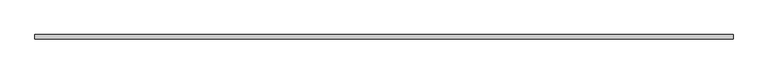
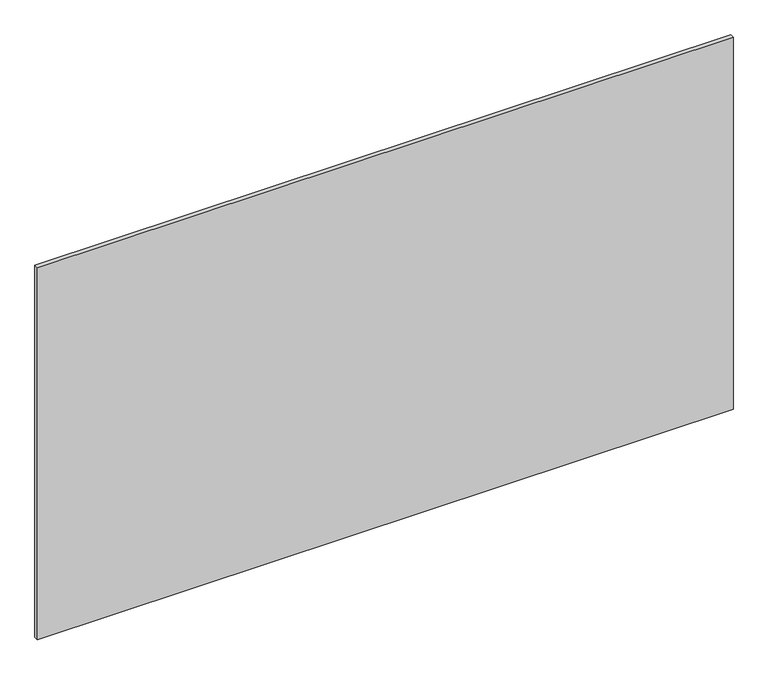
"""IFC4 building model written with IfcOpenShell, lengths in millimetres: railing geometry, ML_Painéis1 : ML_Painéis."""

from ifc_helpers import new_model, si_unit, frame, origin, place, context, project, spatial, polyline, outline, extrude, source, transform, mapped, element, save


def railing_50812a2e(model_context):
    return source(origin(), model_context, "Body", "SweptSolid", [
        extrude(outline(polyline([(-4674.5702584, 2133.3602771), (-4674.5702584, 2121.3602771), (-6620.5702584, 2121.3602771), (-6620.5702584, 2133.3602771), (-4674.5702584, 2133.3602771)])), frame((0.0, 0.0, 4122.0679199), z_axis=(0.0, 0.0, 1.0), x_axis=(1.0, 0.0, 0.0)), (0.0, 0.0, 1.0), 1100.0),
    ])


if __name__ == "__main__":
    model = new_model("IFC4")
    model_context = context("Model", 3, world=origin())
    ifc_project = project(units=[si_unit("LENGTHUNIT", "METRE", prefix="MILLI")], contexts=[model_context])
    site = spatial("IfcSite", under=ifc_project)
    building = spatial("IfcBuilding", under=site)
    placement = place(None, origin())
    railing_shape = railing_50812a2e(model_context)
    element("IfcRailing", 1, ObjectType="ML_Painéis1 : ML_Painéis", at=placement, inside=building, context=model_context, shape_type="MappedRepresentation", body=[
        mapped(railing_shape, transform((0.0, 0.0, 0.0), x_axis=(1.0, 0.0, 0.0), y_axis=(0.0, 1.0, 0.0), z_axis=(0.0, 0.0, 1.0))),
    ])
    save(model, "model.ifc")

# Revit data of these elements
# Type "ML_Painéis1 : ML_Painéis"
#   ME_Área [instance default] = 2.1406 m²
#   ME_Espessura [instance default] = 0.012 m
#   ME_Dist Painéis [instance default] = 0.002 m
#   ME_Compr Painéis [instance default] = 1.946 m
#   ME_Compr [instance default] = 1.95 m
#   ME_Altura [instance default] = 1.10 m
#   ME_Quant Painéis [instance default] = 3
#   ME_Painel Único [instance default] = yes
#   ME_Paineis Vários [instance default] = no
#   ME_Material Tipo Vidro [instance default] = .VIDRO GENÉRICO
# Element 1 (IfcRailing, "ML_Painéis1 : ML_Painéis")
#   Materials on its faces: ".VIDRO GENÉRICO"
# Materials
#   ".VIDRO GENÉRICO": class ".CC_VIDRO", colour RGB 0 128 192, transparency 0.9, Description = "Vidro comum", Cost = 0
